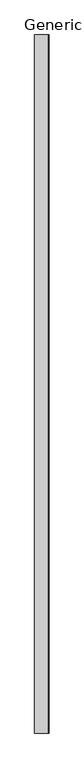
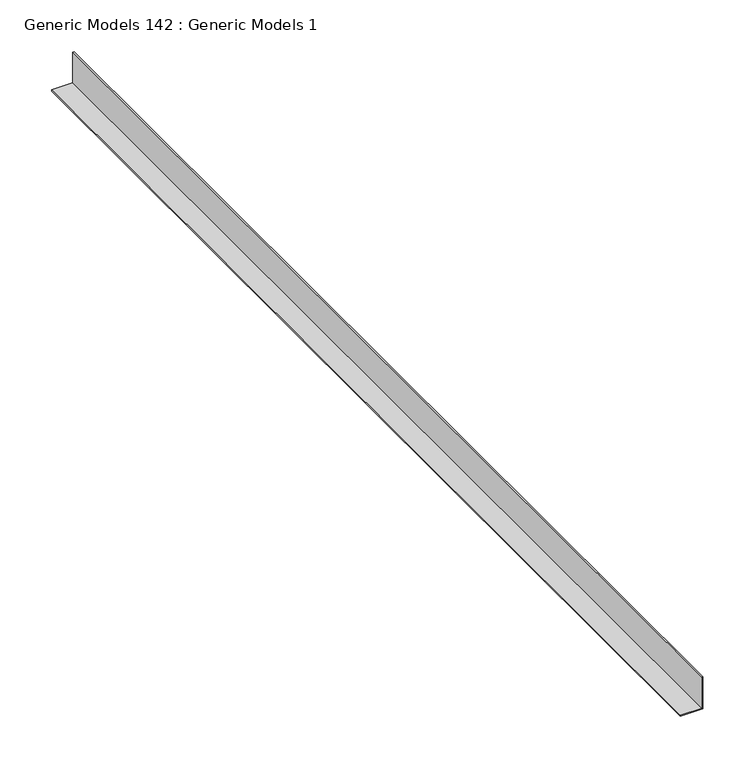
"""IFC4 building model written with IfcOpenShell, lengths in millimetres: proxy geometry, Generic Models 142 : Generic Models 1."""

from ifc_helpers import new_model, si_unit, frame, origin, place, context, project, spatial, polyline, outline, extrude, source, transform, mapped, element, save


def generic_models_142_generic_models_1_dcca0c8b(model_context):
    return source(origin(), model_context, "Body", "SweptSolid", [
        extrude(outline(polyline([(2051.1444308, 46827.9235531), (2051.1444308, 46826.3360531), (2014.6319308, 46826.3360531), (2014.6319308, 46802.5235531), (2013.0444308, 46802.5235531), (2013.0444308, 46827.9235531), (2051.1444308, 46827.9235531)])), frame((0.0, 0.0, 0.0), z_axis=(0.0, 1.0, 0.0), x_axis=(0.0, 0.0, 1.0)), (0.0, 0.0, 1.0), 1219.2),
    ])


if __name__ == "__main__":
    model = new_model("IFC4")
    model_context = context("Model", 3, world=origin())
    ifc_project = project(units=[si_unit("LENGTHUNIT", "METRE", prefix="MILLI")], contexts=[model_context])
    site = spatial("IfcSite", under=ifc_project)
    building = spatial("IfcBuilding", under=site)
    placement = place(None, origin())
    generic_models_142_generic_models_1_shape = generic_models_142_generic_models_1_dcca0c8b(model_context)
    element("IfcBuildingElementProxy", 1, Name="Generic Models 142 : Generic Models 1", ObjectType="Generic Models 142 : Generic Models 1", at=placement, inside=building, context=model_context, shape_type="MappedRepresentation", body=[
        mapped(generic_models_142_generic_models_1_shape, transform((0.0, 0.0, 0.0), x_axis=(1.0, 0.0, 0.0), y_axis=(0.0, 1.0, 0.0), z_axis=(0.0, 0.0, 1.0))),
    ])
    save(model, "model.ifc")

# Revit data of these elements
# Element 1 (IfcBuildingElementProxy, "Generic Models 142 : Generic Models 1")
#   Materials on its faces: "CEILING TRACK TO MATCH EXISTING"
# Materials
#   "CEILING TRACK TO MATCH EXISTING": class "Unassigned", colour RGB 210 209 208, transparency 0, Keynote = "M05121300.02", Cost = 0
